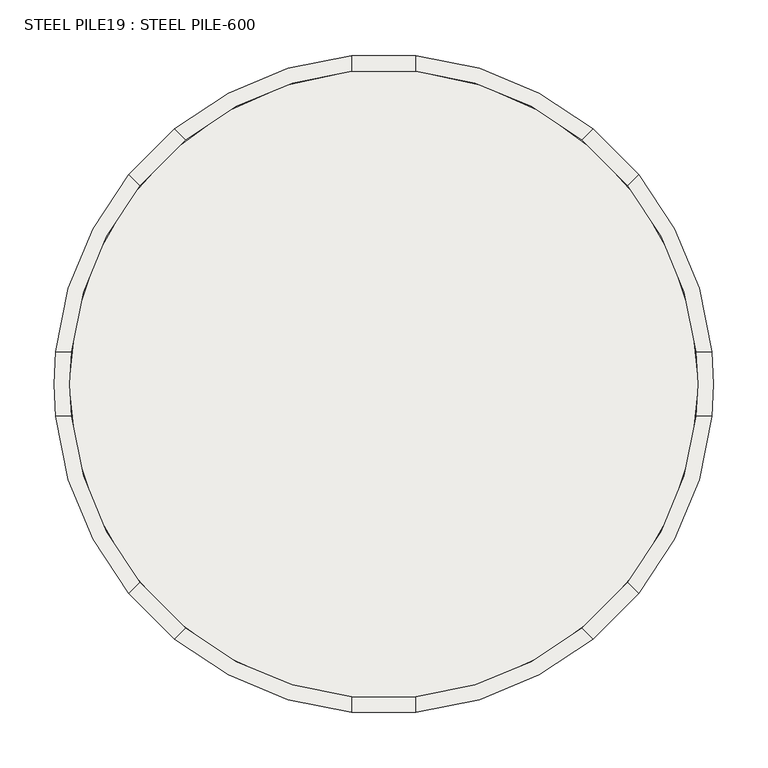
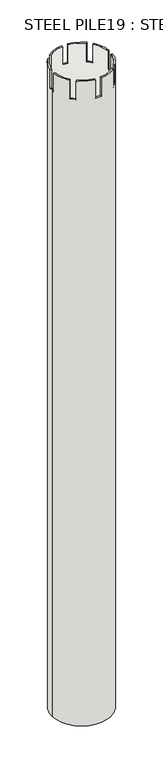
"""IFC4 building model written with IfcOpenShell, lengths in millimetres: slab geometry, STEEL PILE19 : STEEL PILE-600."""

from ifc_helpers import new_model, si_unit, point, frame, frame_2d, origin, place, context, project, spatial, polyline, circle_curve, trimmed, segment, composite_curve, outline, extrude, source, transform, mapped, element, save
from ifc_brep_helpers import plane_surface, cylinder_surface, revolved_surface, advanced_brep


def steel_pile19_steel_pile_600_0419001b(model_context):
    return source(origin(), model_context, "Body", "SolidModel", [
        advanced_brep(
        [(7615.5, 33979.5208589, -7500.0), (8224.5, 33979.5208589, -7500.0), (7629.5, 33979.5208589, -7500.0), (8210.5, 33979.5208589, -7500.0), (8155.4796847, 33786.467581, -500.0), (8223.0185638, 33949.5208589, -500.0), (8208.9467944, 33949.5208589, -500.0), (8145.5294412, 33796.4178246, -500.0), (7950.0, 33676.5022951, -500.0), (8113.0532778, 33744.0411742, -500.0), (8103.1030343, 33753.9914177, -500.0), (7950.0, 33690.5740645, -500.0), (7726.9467222, 33744.0411742, -500.0), (7890.0, 33676.5022951, -500.0), (7890.0, 33690.5740645, -500.0), (7736.8969657, 33753.9914177, -500.0), (7616.9814362, 33949.5208589, -500.0), (7684.5203153, 33786.467581, -500.0), (7694.4705588, 33796.4178246, -500.0), (7631.0532056, 33949.5208589, -500.0), (7684.5203153, 34172.5741367, -500.0), (7616.9814362, 34009.5208589, -500.0), (7631.0532056, 34009.5208589, -500.0), (7694.4705588, 34162.6238932, -500.0), (7890.0, 34282.5394227, -500.0), (7726.9467222, 34215.0005436, -500.0), (7736.8969657, 34205.0503001, -500.0), (7890.0, 34268.4676533, -500.0), (8113.0532778, 34215.0005436, -500.0), (7950.0, 34282.5394227, -500.0), (7950.0, 34268.4676533, -500.0), (8103.1030343, 34205.0503001, -500.0), (8223.0185638, 34009.5208589, -500.0), (8155.4796847, 34172.5741367, -500.0), (8145.5294412, 34162.6238932, -500.0), (8208.9467944, 34009.5208589, -500.0), (8224.5, 33979.5208589, -700.0), (8223.0185638, 33949.5208589, -700.0), (8155.4796847, 33786.467581, -700.0), (8113.0532778, 33744.0411742, -700.0), (7950.0, 33676.5022951, -700.0), (7890.0, 33676.5022951, -700.0), (7726.9467222, 33744.0411742, -700.0), (7684.5203153, 33786.467581, -700.0), (7616.9814362, 33949.5208589, -700.0), (7615.5, 33979.5208589, -700.0), (7616.9814362, 34009.5208589, -700.0), (7684.5203153, 34172.5741367, -700.0), (7726.9467222, 34215.0005436, -700.0), (7890.0, 34282.5394227, -700.0), (7950.0, 34282.5394227, -700.0), (8113.0532778, 34215.0005436, -700.0), (8155.4796847, 34172.5741367, -700.0), (8223.0185638, 34009.5208589, -700.0), (8210.5, 33979.5208589, -700.0), (8208.9467944, 34009.5208589, -700.0), (8145.5294412, 34162.6238932, -700.0), (8103.1030343, 34205.0503001, -700.0), (7950.0, 34268.4676533, -700.0), (7890.0, 34268.4676533, -700.0), (7736.8969657, 34205.0503001, -700.0), (7694.4705588, 34162.6238932, -700.0), (7631.0532056, 34009.5208589, -700.0), (7629.5, 33979.5208589, -700.0), (7631.0532056, 33949.5208589, -700.0), (7694.4705588, 33796.4178246, -700.0), (7736.8969657, 33753.9914177, -700.0), (7890.0, 33690.5740645, -700.0), (7950.0, 33690.5740645, -700.0), (8103.1030343, 33753.9914177, -700.0), (8145.5294412, 33796.4178246, -700.0), (8208.9467944, 33949.5208589, -700.0)],
        [
            (0, 1, circle_curve(frame((7920.0, 33979.5208589, -7500.0), z_axis=(0.0, 0.0, -1.0), x_axis=(1.0, 0.0, 0.0)), 304.5)),
            (1, 0, circle_curve(frame((7920.0, 33979.5208589, -7500.0), z_axis=(0.0, 0.0, -1.0), x_axis=(1.0, 0.0, 0.0)), 304.5)),
            (2, 3, circle_curve(frame((7920.0, 33979.5208589, -7500.0), z_axis=(0.0, 0.0, 1.0), x_axis=(1.0, 0.0, 0.0)), 290.5)),
            (3, 2, circle_curve(frame((7920.0, 33979.5208589, -7500.0), z_axis=(0.0, 0.0, 1.0), x_axis=(1.0, 0.0, 0.0)), 290.5)),
            (4, 5, circle_curve(frame((7920.0, 33979.5208589, -500.0), z_axis=(0.0, 0.0, 1.0), x_axis=(1.0, 0.0, 0.0)), 304.5)),
            (5, 6),
            (6, 7, circle_curve(frame((7920.0, 33979.5208589, -500.0), z_axis=(0.0, 0.0, -1.0), x_axis=(1.0, 0.0, 0.0)), 290.5)),
            (7, 4),
            (8, 9, circle_curve(frame((7920.0, 33979.5208589, -500.0), z_axis=(0.0, 0.0, 1.0), x_axis=(1.0, 0.0, 0.0)), 304.5)),
            (9, 10),
            (10, 11, circle_curve(frame((7920.0, 33979.5208589, -500.0), z_axis=(0.0, 0.0, -1.0), x_axis=(1.0, 0.0, 0.0)), 290.5)),
            (11, 8),
            (12, 13, circle_curve(frame((7920.0, 33979.5208589, -500.0), z_axis=(0.0, 0.0, 1.0), x_axis=(1.0, 0.0, 0.0)), 304.5)),
            (13, 14),
            (14, 15, circle_curve(frame((7920.0, 33979.5208589, -500.0), z_axis=(0.0, 0.0, -1.0), x_axis=(1.0, 0.0, 0.0)), 290.5)),
            (15, 12),
            (16, 17, circle_curve(frame((7920.0, 33979.5208589, -500.0), z_axis=(0.0, 0.0, 1.0), x_axis=(1.0, 0.0, 0.0)), 304.5)),
            (17, 18),
            (18, 19, circle_curve(frame((7920.0, 33979.5208589, -500.0), z_axis=(0.0, 0.0, -1.0), x_axis=(1.0, 0.0, 0.0)), 290.5)),
            (19, 16),
            (20, 21, circle_curve(frame((7920.0, 33979.5208589, -500.0), z_axis=(0.0, 0.0, 1.0), x_axis=(1.0, 0.0, 0.0)), 304.5)),
            (21, 22),
            (22, 23, circle_curve(frame((7920.0, 33979.5208589, -500.0), z_axis=(0.0, 0.0, -1.0), x_axis=(1.0, 0.0, 0.0)), 290.5)),
            (23, 20),
            (24, 25, circle_curve(frame((7920.0, 33979.5208589, -500.0), z_axis=(0.0, 0.0, 1.0), x_axis=(1.0, 0.0, 0.0)), 304.5)),
            (25, 26),
            (26, 27, circle_curve(frame((7920.0, 33979.5208589, -500.0), z_axis=(0.0, 0.0, -1.0), x_axis=(1.0, 0.0, 0.0)), 290.5)),
            (27, 24),
            (28, 29, circle_curve(frame((7920.0, 33979.5208589, -500.0), z_axis=(0.0, 0.0, 1.0), x_axis=(1.0, 0.0, 0.0)), 304.5)),
            (29, 30),
            (30, 31, circle_curve(frame((7920.0, 33979.5208589, -500.0), z_axis=(0.0, 0.0, -1.0), x_axis=(1.0, 0.0, 0.0)), 290.5)),
            (31, 28),
            (32, 33, circle_curve(frame((7920.0, 33979.5208589, -500.0), z_axis=(0.0, 0.0, 1.0), x_axis=(1.0, 0.0, 0.0)), 304.5)),
            (33, 34),
            (34, 35, circle_curve(frame((7920.0, 33979.5208589, -500.0), z_axis=(0.0, 0.0, -1.0), x_axis=(1.0, 0.0, 0.0)), 290.5)),
            (35, 32),
            (1, 36),
            (36, 37, circle_curve(frame((7920.0, 33979.5208589, -700.0), z_axis=(0.0, 0.0, -1.0), x_axis=(1.0, 0.0, 0.0)), 304.5)),
            (37, 5),
            (4, 38),
            (38, 39, circle_curve(frame((7920.0, 33979.5208589, -700.0), z_axis=(0.0, 0.0, -1.0), x_axis=(1.0, 0.0, 0.0)), 304.5)),
            (39, 9),
            (8, 40),
            (40, 41, circle_curve(frame((7920.0, 33979.5208589, -700.0), z_axis=(0.0, 0.0, -1.0), x_axis=(1.0, 0.0, 0.0)), 304.5)),
            (41, 13),
            (12, 42),
            (42, 43, circle_curve(frame((7920.0, 33979.5208589, -700.0), z_axis=(0.0, 0.0, -1.0), x_axis=(1.0, 0.0, 0.0)), 304.5)),
            (43, 17),
            (16, 44),
            (44, 45, circle_curve(frame((7920.0, 33979.5208589, -700.0), z_axis=(0.0, 0.0, -1.0), x_axis=(1.0, 0.0, 0.0)), 304.5)),
            (45, 0),
            (45, 46, circle_curve(frame((7920.0, 33979.5208589, -700.0), z_axis=(0.0, 0.0, -1.0), x_axis=(1.0, 0.0, 0.0)), 304.5)),
            (46, 21),
            (20, 47),
            (47, 48, circle_curve(frame((7920.0, 33979.5208589, -700.0), z_axis=(0.0, 0.0, -1.0), x_axis=(1.0, 0.0, 0.0)), 304.5)),
            (48, 25),
            (24, 49),
            (49, 50, circle_curve(frame((7920.0, 33979.5208589, -700.0), z_axis=(0.0, 0.0, -1.0), x_axis=(1.0, 0.0, 0.0)), 304.5)),
            (50, 29),
            (28, 51),
            (51, 52, circle_curve(frame((7920.0, 33979.5208589, -700.0), z_axis=(0.0, 0.0, -1.0), x_axis=(1.0, 0.0, 0.0)), 304.5)),
            (52, 33),
            (32, 53),
            (53, 36, circle_curve(frame((7920.0, 33979.5208589, -700.0), z_axis=(0.0, 0.0, -1.0), x_axis=(1.0, 0.0, 0.0)), 304.5)),
            (3, 54),
            (54, 55, circle_curve(frame((7920.0, 33979.5208589, -700.0), z_axis=(0.0, 0.0, 1.0), x_axis=(1.0, 0.0, 0.0)), 290.5)),
            (55, 35),
            (34, 56),
            (56, 57, circle_curve(frame((7920.0, 33979.5208589, -700.0), z_axis=(0.0, 0.0, 1.0), x_axis=(1.0, 0.0, 0.0)), 290.5)),
            (57, 31),
            (30, 58),
            (58, 59, circle_curve(frame((7920.0, 33979.5208589, -700.0), z_axis=(0.0, 0.0, 1.0), x_axis=(1.0, 0.0, 0.0)), 290.5)),
            (59, 27),
            (26, 60),
            (60, 61, circle_curve(frame((7920.0, 33979.5208589, -700.0), z_axis=(0.0, 0.0, 1.0), x_axis=(1.0, 0.0, 0.0)), 290.5)),
            (61, 23),
            (22, 62),
            (62, 63, circle_curve(frame((7920.0, 33979.5208589, -700.0), z_axis=(0.0, 0.0, 1.0), x_axis=(1.0, 0.0, 0.0)), 290.5)),
            (63, 2),
            (63, 64, circle_curve(frame((7920.0, 33979.5208589, -700.0), z_axis=(0.0, 0.0, 1.0), x_axis=(1.0, 0.0, 0.0)), 290.5)),
            (64, 19),
            (18, 65),
            (65, 66, circle_curve(frame((7920.0, 33979.5208589, -700.0), z_axis=(0.0, 0.0, 1.0), x_axis=(1.0, 0.0, 0.0)), 290.5)),
            (66, 15),
            (14, 67),
            (67, 68, circle_curve(frame((7920.0, 33979.5208589, -700.0), z_axis=(0.0, 0.0, 1.0), x_axis=(1.0, 0.0, 0.0)), 290.5)),
            (68, 11),
            (10, 69),
            (69, 70, circle_curve(frame((7920.0, 33979.5208589, -700.0), z_axis=(0.0, 0.0, 1.0), x_axis=(1.0, 0.0, 0.0)), 290.5)),
            (70, 7),
            (6, 71),
            (71, 54, circle_curve(frame((7920.0, 33979.5208589, -700.0), z_axis=(0.0, 0.0, 1.0), x_axis=(1.0, 0.0, 0.0)), 290.5)),
            (65, 43),
            (42, 66),
            (67, 41),
            (40, 68),
            (69, 39),
            (38, 70),
            (71, 37),
            (53, 55),
            (56, 52),
            (51, 57),
            (58, 50),
            (49, 59),
            (60, 48),
            (47, 61),
            (62, 46),
            (44, 64),
        ],
        [
            plane_surface(frame((8224.5, 33979.5208589, -7500.0), z_axis=(0.0, 0.0, -1.0), x_axis=(0.0, -1.0, 0.0))),
            plane_surface(frame((8224.5, 33979.5208589, -500.0), z_axis=(0.0, 0.0, 1.0), x_axis=(0.0, 1.0, 0.0))),
            cylinder_surface(frame((7920.0, 33979.5208589, -7500.0), z_axis=(0.0, 0.0, 1.0), x_axis=(1.0, 0.0, 0.0)), 304.5),
            revolved_surface(polyline([(8210.5, 33979.5208589, -7500.0), (8210.5, 33979.5208589, -500.0)]), (7920.0, 33979.5208589, 200.0), (0.0, 0.0, -1.0)),
            plane_surface(frame((7450.0, 33949.5208589, -700.0), z_axis=(0.0, 0.0, 1.0), x_axis=(-1.0, 0.0, 0.0))),
            plane_surface(frame((7847.5735931, 33949.5208589, -700.0), z_axis=(0.0, 1.0, 0.0), x_axis=(0.0, 0.0, 1.0))),
            plane_surface(frame((7450.0, 34009.5208589, -700.0), z_axis=(0.0, -1.0, 0.0), x_axis=(0.0, 0.0, 1.0))),
            plane_surface(frame((7847.5735931, 34009.5208589, -700.0), z_axis=(0.7071067811865516, 0.7071067811865435, 0.0), x_axis=(0.0, 0.0, 1.0))),
            plane_surface(frame((7608.8730163, 34333.0742495, -700.0), z_axis=(-0.707106781186553, -0.7071067811865421, 0.0), x_axis=(0.0, 0.0, 1.0))),
            plane_surface(frame((7890.0, 34051.9472658, -700.0), z_axis=(1.0, 0.0, 0.0), x_axis=(0.0, 0.0, 1.0))),
            plane_surface(frame((7950.0, 34449.5208589, -700.0), z_axis=(-1.0, 0.0, 0.0), x_axis=(0.0, 0.0, 1.0))),
            plane_surface(frame((7950.0, 34051.9472658, -700.0), z_axis=(0.7071067811865516, -0.7071067811865435, 0.0), x_axis=(0.0, 0.0, 1.0))),
            plane_surface(frame((8273.5533906, 34290.6478426, -700.0), z_axis=(-0.7071067811865448, 0.7071067811865502, 0.0), x_axis=(0.0, 0.0, 1.0))),
            plane_surface(frame((7992.4264069, 34009.5208589, -700.0), z_axis=(0.0, -1.0, 0.0), x_axis=(0.0, 0.0, 1.0))),
            plane_surface(frame((8390.0, 33949.5208589, -700.0), z_axis=(0.0, 1.0, 0.0), x_axis=(0.0, 0.0, 1.0))),
            plane_surface(frame((7992.4264069, 33949.5208589, -700.0), z_axis=(-0.7071067811865489, -0.7071067811865462, 0.0), x_axis=(0.0, 0.0, 1.0))),
            plane_surface(frame((8231.1269837, 33625.9674683, -700.0), z_axis=(0.7071067811865462, 0.7071067811865489, 0.0), x_axis=(0.0, 0.0, 1.0))),
            plane_surface(frame((7950.0, 33907.094452, -700.0), z_axis=(-1.0, 0.0, 0.0), x_axis=(0.0, 0.0, 1.0))),
            plane_surface(frame((7890.0, 33509.5208589, -700.0), z_axis=(1.0, 0.0, 0.0), x_axis=(0.0, 0.0, 1.0))),
            plane_surface(frame((7890.0, 33907.094452, -700.0), z_axis=(-0.7071067811865516, 0.7071067811865435, 0.0), x_axis=(0.0, 0.0, 1.0))),
            plane_surface(frame((7566.4466094, 33668.3938752, -700.0), z_axis=(0.7071067811865448, -0.7071067811865502, 0.0), x_axis=(0.0, 0.0, 1.0))),
        ],
        [
            (0, [[1, 2], [3, 4]]),
            (1, [[5, 6, 7, 8]]),
            (1, [[9, 10, 11, 12]]),
            (1, [[13, 14, 15, 16]]),
            (1, [[17, 18, 19, 20]]),
            (1, [[21, 22, 23, 24]]),
            (1, [[25, 26, 27, 28]]),
            (1, [[29, 30, 31, 32]]),
            (1, [[33, 34, 35, 36]]),
            (2, [[-2, 37, 38, 39, -5, 40, 41, 42, -9, 43, 44, 45, -13, 46, 47, 48, -17, 49, 50, 51]]),
            (2, [[-1, -51, 52, 53, -21, 54, 55, 56, -25, 57, 58, 59, -29, 60, 61, 62, -33, 63, 64, -37]]),
            (3, [[-4, 65, 66, 67, -35, 68, 69, 70, -31, 71, 72, 73, -27, 74, 75, 76, -23, 77, 78, 79]]),
            (3, [[-3, -79, 80, 81, -19, 82, 83, 84, -15, 85, 86, 87, -11, 88, 89, 90, -7, 91, 92, -65]]),
            (4, [[93, -47, 94, -83]]),
            (4, [[95, -44, 96, -86]]),
            (4, [[97, -41, 98, -89]]),
            (4, [[99, -38, -64, 100, -66, -92]]),
            (4, [[101, -61, 102, -69]]),
            (4, [[103, -58, 104, -72]]),
            (4, [[105, -55, 106, -75]]),
            (4, [[107, -52, -50, 108, -80, -78]]),
            (5, [[-108, -49, -20, -81]]),
            (6, [[-107, -77, -22, -53]]),
            (7, [[-106, -54, -24, -76]]),
            (8, [[-105, -74, -26, -56]]),
            (9, [[-104, -57, -28, -73]]),
            (10, [[-103, -71, -30, -59]]),
            (11, [[-102, -60, -32, -70]]),
            (12, [[-101, -68, -34, -62]]),
            (13, [[-100, -63, -36, -67]]),
            (14, [[-99, -91, -6, -39]]),
            (15, [[-98, -40, -8, -90]]),
            (16, [[-97, -88, -10, -42]]),
            (17, [[-96, -43, -12, -87]]),
            (18, [[-95, -85, -14, -45]]),
            (19, [[-94, -46, -16, -84]]),
            (20, [[-93, -82, -18, -48]]),
        ],
    ),
        extrude(outline(composite_curve([segment(trimmed(circle_curve(frame_2d((7920.0, 33979.5208589)), 290.5), [point((7629.5, 33979.5208589))], [point((8210.5, 33979.5208589))], False, "CARTESIAN"), True, "CONTINUOUS"), segment(trimmed(circle_curve(frame_2d((7920.0, 33979.5208589)), 290.5), [point((8210.5, 33979.5208589))], [point((7629.5, 33979.5208589))], False, "CARTESIAN"), True, "CONTINUOUS")], self_intersect=False)), frame((0.0, 0.0, -2530.0), z_axis=(0.0, 0.0, 1.0), x_axis=(1.0, 0.0, 0.0)), (0.0, 0.0, 1.0), 30.0),
    ])


if __name__ == "__main__":
    model = new_model("IFC4")
    model_context = context("Model", 3, world=origin())
    ifc_project = project(units=[si_unit("LENGTHUNIT", "METRE", prefix="MILLI")], contexts=[model_context])
    site = spatial("IfcSite", under=ifc_project)
    building = spatial("IfcBuilding", under=site)
    placement = place(None, origin())
    steel_pile19_steel_pile_600_shape = steel_pile19_steel_pile_600_0419001b(model_context)
    element("IfcSlab", 1, ObjectType="STEEL PILE19 : STEEL PILE-600", at=placement, inside=building, context=model_context, shape_type="MappedRepresentation", body=[
        mapped(steel_pile19_steel_pile_600_shape, transform((0.0, 0.0, 0.0), x_axis=(1.0, 0.0, 0.0), y_axis=(0.0, 1.0, 0.0), z_axis=(0.0, 0.0, 1.0))),
    ])
    save(model, "model.ifc")

# Revit data of these elements
# Element 1 (IfcSlab, "STEEL PILE19 : STEEL PILE-600")
#   Materials on its faces: "Metal - Steel"
# Materials
#   "Metal - Steel": class "Metal", colour RGB 247 247 247, transparency 0, Cost = 0
